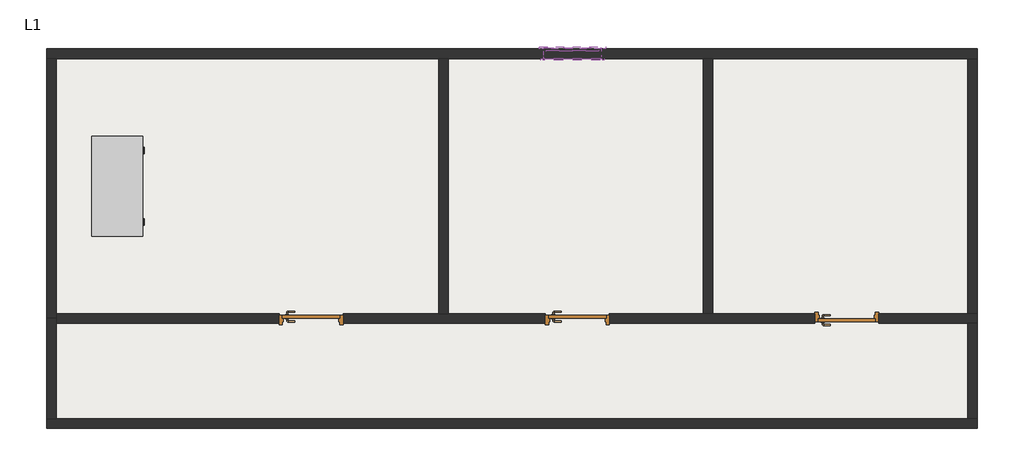
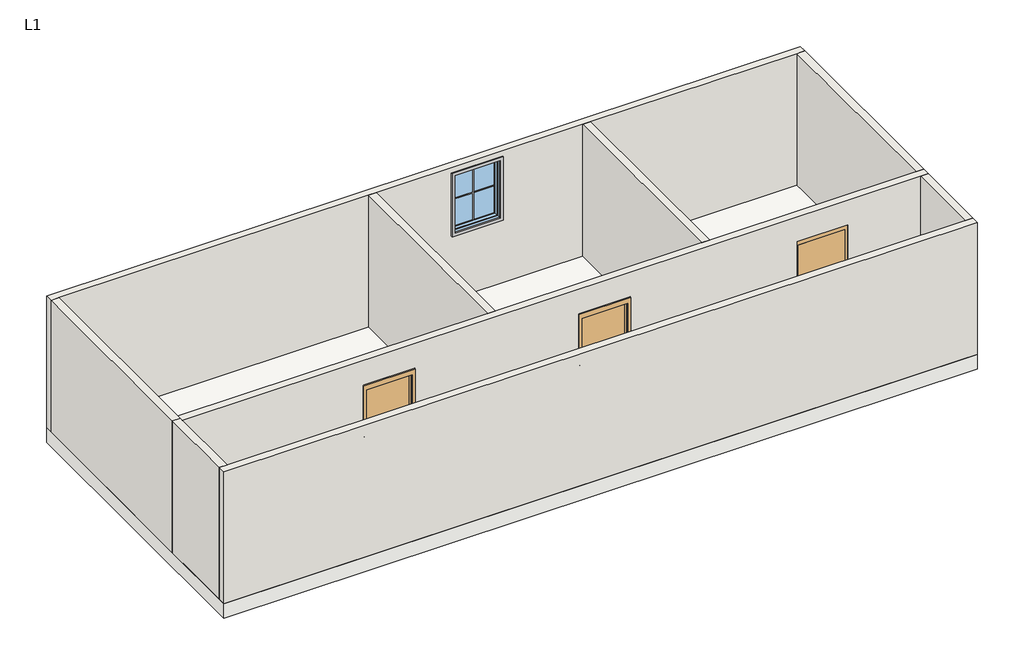
# One storey: 9 walls, 3 doors, 3 proxies, 1 furniture element, 1 slab, 1 window.
"""IFC4 building model written with IfcOpenShell, lengths in millimetres."""

import ifcopenshell
import ifcopenshell.guid

model = None  # the IFC model being written
_history = None  # IfcOwnerHistory: only IFC2X3 demands one
_inside = {}  # id of a spatial element -> (the spatial element, [elements in it])
_under = {}  # id of a project, library or spatial element -> (it, [spatial elements below it])
_declared = {}  # id of a project -> (the project, [libraries it declares])
_typed = {}  # id of a type object -> (the type object, [elements of that type])
_made_of = {}  # id of a material, layer set ... -> (it, [elements and type objects made of it])


def new_model(schema):
    """Start an empty IFC model of exactly this schema.

    Asked for "IFC4X3", IfcOpenShell would pick the latest addendum, in which some entities
    have other attributes; the version numbers below select the first issue.
    IFC2X3 requires an IfcOwnerHistory on every rooted entity: one is made here for all.
    """
    global model, _history
    if schema == "IFC4X3":
        model = ifcopenshell.file(schema_version=(4, 3, 0, 0))
    else:
        model = ifcopenshell.file(schema=schema)
    _inside.clear()
    _under.clear()
    _declared.clear()
    _typed.clear()
    _made_of.clear()
    _history = None
    if model.schema == "IFC2X3":
        org = make("IfcOrganization", Name="unknown")
        user = make(
            "IfcPersonAndOrganization",
            ThePerson=make("IfcPerson", FamilyName="unknown"),
            TheOrganization=org,
        )
        app = make(
            "IfcApplication",
            ApplicationDeveloper=org,
            Version="unknown",
            ApplicationFullName="unknown",
            ApplicationIdentifier="unknown",
        )
        _history = make(
            "IfcOwnerHistory",
            OwningUser=user,
            OwningApplication=app,
            ChangeAction="ADDED",
            CreationDate=0,
        )
    return model


def make(cls, **values):
    """One entity of the class cls with the attributes given. An attribute that is None is left unset."""
    return model.create_entity(
        cls, **{name: value for name, value in values.items() if value is not None}
    )


def rooted(cls, **values):
    """An entity with a GlobalId (a new one), such as an element, a storey or a relation."""
    return make(cls, GlobalId=ifcopenshell.guid.new(), OwnerHistory=_history, **values)


def si_unit(unit_type, name, prefix=None):
    """IfcSIUnit, for example si_unit("LENGTHUNIT", "METRE", prefix="MILLI")."""
    return make("IfcSIUnit", UnitType=unit_type, Prefix=prefix, Name=name)


def assignment(units):
    """IfcUnitAssignment: the units of a project."""
    return None if units is None else make("IfcUnitAssignment", Units=units)


def point(xyz):
    """IfcCartesianPoint."""
    return None if xyz is None else make("IfcCartesianPoint", Coordinates=xyz)


def direction(xyz):
    """IfcDirection."""
    return None if xyz is None else make("IfcDirection", DirectionRatios=xyz)


def frame(location, z_axis=None, x_axis=None):
    """IfcAxis2Placement3D, a coordinate frame: its origin and axes. An axis left out is left unset."""
    return make(
        "IfcAxis2Placement3D",
        Location=point(location),
        Axis=direction(z_axis),
        RefDirection=direction(x_axis),
    )


def frame_2d(location, x_axis=None):
    """IfcAxis2Placement2D, a coordinate frame in the plane: its origin and x axis."""
    return make(
        "IfcAxis2Placement2D", Location=point(location), RefDirection=direction(x_axis)
    )


def origin():
    """The frame at (0, 0, 0) with its axes left unset."""
    return frame((0.0, 0.0, 0.0))


def origin_with_axes():
    """The frame at (0, 0, 0) with the z axis (0, 0, 1) and the x axis (1, 0, 0) written out."""
    return frame((0.0, 0.0, 0.0), z_axis=(0.0, 0.0, 1.0), x_axis=(1.0, 0.0, 0.0))


def place(relative_to, where):
    """IfcLocalPlacement: puts the frame where relative to a parent placement (None: the world)."""
    return make(
        "IfcLocalPlacement", PlacementRelTo=relative_to, RelativePlacement=where
    )


def context(
    kind, dimensions, precision=None, world=None, true_north=None, identifier=None
):
    """IfcGeometricRepresentationContext, for example the 3D "Model" context."""
    return make(
        "IfcGeometricRepresentationContext",
        ContextIdentifier=identifier,
        ContextType=kind,
        CoordinateSpaceDimension=dimensions,
        Precision=precision,
        WorldCoordinateSystem=world,
        TrueNorth=true_north,
    )


def project(units=None, contexts=None):
    """IfcProject with its units and contexts."""
    return rooted(
        "IfcProject",
        Name="project",
        RepresentationContexts=contexts,
        UnitsInContext=assignment(units),
    )


def spatial(cls, under=None, at=None, **own):
    """A site, building, storey or space (cls), placed at a placement, below another one or the project."""
    s = rooted(cls, ObjectPlacement=at, **own)
    if under is not None:
        _under.setdefault(under.id(), (under, []))[1].append(s)
    return s


def polyline(points):
    """IfcPolyline through the points."""
    return make("IfcPolyline", Points=[point(p) for p in points])


def circle_curve(where, radius):
    """IfcCircle in the frame where."""
    return make("IfcCircle", Position=where, Radius=radius)


def ellipse_curve(where, semi_axis1, semi_axis2):
    """IfcEllipse in the frame where."""
    return make(
        "IfcEllipse", Position=where, SemiAxis1=semi_axis1, SemiAxis2=semi_axis2
    )


def trimmed(basis, trim1, trim2, sense, master):
    """IfcTrimmedCurve: the piece of a basis curve between two trims."""
    return make(
        "IfcTrimmedCurve",
        BasisCurve=basis,
        Trim1=trim1,
        Trim2=trim2,
        SenseAgreement=sense,
        MasterRepresentation=master,
    )


def segment(curve, same_sense, transition):
    """IfcCompositeCurveSegment."""
    return make(
        "IfcCompositeCurveSegment",
        Transition=transition,
        SameSense=same_sense,
        ParentCurve=curve,
    )


def composite_curve(segments, self_intersect=None):
    """IfcCompositeCurve: segments joined end to end."""
    return make("IfcCompositeCurve", Segments=segments, SelfIntersect=self_intersect)


def outline(outer, holes=None, kind="AREA"):
    """IfcArbitraryClosedProfileDef: a profile drawn as a closed curve; with holes, ...WithVoids."""
    if holes is None:
        return make("IfcArbitraryClosedProfileDef", ProfileType=kind, OuterCurve=outer)
    return make(
        "IfcArbitraryProfileDefWithVoids",
        ProfileType=kind,
        OuterCurve=outer,
        InnerCurves=holes,
    )


def extrude(swept, where, along, depth):
    """IfcExtrudedAreaSolid: the profile swept, set in the frame where, extruded along a direction by depth."""
    return make(
        "IfcExtrudedAreaSolid",
        SweptArea=swept,
        Position=where,
        ExtrudedDirection=direction(along),
        Depth=depth,
    )


def faces_of(points, faces, orient=None, outer=None):
    """IfcFace entities. A face is a list of loops; a loop is a list of indices into points, from 0.

    orient and outer hold one flag for each loop. By default every Orientation is true, the
    first loop of a face is its IfcFaceOuterBound and the others are IfcFaceBound.
    """
    made = []
    for i, loops in enumerate(faces):
        bounds = []
        for j, loop in enumerate(loops):
            is_outer = j == 0 if outer is None else outer[i][j]
            bounds.append(
                make(
                    "IfcFaceOuterBound" if is_outer else "IfcFaceBound",
                    Bound=make("IfcPolyLoop", Polygon=[points[k] for k in loop]),
                    Orientation=True if orient is None else orient[i][j],
                )
            )
        made.append(make("IfcFace", Bounds=bounds))
    return made


def faceted_brep(points, faces, orient=None, outer=None, voids=None):
    """IfcFacetedBrep: a solid bounded by flat faces; with voids (closed shells), ...WithVoids."""
    shared = [point(p) for p in points]
    hull = make("IfcClosedShell", CfsFaces=faces_of(shared, faces, orient, outer))
    if voids is None:
        return make("IfcFacetedBrep", Outer=hull)
    return make(
        "IfcFacetedBrepWithVoids",
        Outer=hull,
        Voids=[
            make(cls, CfsFaces=faces_of(shared, fs, o, b)) for cls, fs, o, b in voids
        ],
    )


def shape(context_of_items, identifier, shape_type, items):
    """IfcShapeRepresentation: the items that make up one representation, for example the "Body"."""
    return make(
        "IfcShapeRepresentation",
        ContextOfItems=context_of_items,
        RepresentationIdentifier=identifier,
        RepresentationType=shape_type,
        Items=items,
    )


def source(mapping_origin, context_of_items, identifier, shape_type, items):
    """IfcRepresentationMap: a shape defined once, which mapped items show again and again."""
    return make(
        "IfcRepresentationMap",
        MappingOrigin=mapping_origin,
        MappedRepresentation=shape(context_of_items, identifier, shape_type, items),
    )


def transform(
    local_origin,
    x_axis=None,
    y_axis=None,
    z_axis=None,
    scale=None,
    scale2=None,
    scale3=None,
    uniform=True,
):
    """IfcCartesianTransformationOperator3D, or its non-uniform kind. x_axis, y_axis, z_axis: its Axis1, 2, 3."""
    if uniform:
        return make(
            "IfcCartesianTransformationOperator3D",
            Axis1=direction(x_axis),
            Axis2=direction(y_axis),
            LocalOrigin=point(local_origin),
            Scale=scale,
            Axis3=direction(z_axis),
        )
    return make(
        "IfcCartesianTransformationOperator3DnonUniform",
        Axis1=direction(x_axis),
        Axis2=direction(y_axis),
        LocalOrigin=point(local_origin),
        Scale=scale,
        Axis3=direction(z_axis),
        Scale2=scale2,
        Scale3=scale3,
    )


def mapped(mapping_source, mapping_target):
    """IfcMappedItem: shows the shape of a source again, moved by a transform."""
    return make(
        "IfcMappedItem", MappingSource=mapping_source, MappingTarget=mapping_target
    )


def made_of(thing, what):
    """Note that an element or type object is made of a material, layer set ...; save() writes the relation."""
    if what is not None:
        _made_of.setdefault(what.id(), (what, []))[1].append(thing)
    return thing


def element(
    cls,
    number,
    at=None,
    inside=None,
    cuts=None,
    type_object=None,
    material=None,
    context=None,
    identifier="Body",
    shape_type=None,
    held_by="IfcProductDefinitionShape",
    body=None,
    shapes=None,
    **own,
):
    """One element of the class cls, such as IfcWall. Its Tag is "e" and its number.

    at: its placement. inside: the storey or other place that contains it. cuts: it is an
    opening in that element (IfcRelVoidsElement). A single representation is given by context,
    identifier, shape_type and body (its items); several are given by shapes. held_by: the class
    of the entity that holds the representations. save() writes the other relations.
    """
    e = rooted(cls, Tag="e%d" % number, ObjectPlacement=at, **own)
    if body is not None:
        shapes = [shape(context, identifier, shape_type, body)]
    if shapes is not None:
        e.Representation = make(held_by, Representations=shapes)
    if inside is not None:
        _inside.setdefault(inside.id(), (inside, []))[1].append(e)
    if cuts is not None:
        rooted(
            "IfcRelVoidsElement", RelatingBuildingElement=cuts, RelatedOpeningElement=e
        )
    if type_object is not None:
        _typed.setdefault(type_object.id(), (type_object, []))[1].append(e)
    return made_of(e, material)


def aggregate(whole, parts):
    """IfcRelAggregates: a whole, such as a stair, and the parts it consists of."""
    return rooted("IfcRelAggregates", RelatingObject=whole, RelatedObjects=parts)


def save(model, path):
    """Write the relations noted so far, then the file.

    IfcRelAggregates (storeys below a building ...), IfcRelContainedInSpatialStructure (elements
    in a storey), IfcRelDefinesByType, IfcRelAssociatesMaterial and IfcRelDeclares: one each for
    every whole, place, type object, material and project.
    """
    for whole, parts in _under.values():
        aggregate(whole, parts)
    for where, things in _inside.values():
        rooted(
            "IfcRelContainedInSpatialStructure",
            RelatedElements=things,
            RelatingStructure=where,
        )
    for kind, things in _typed.values():
        rooted("IfcRelDefinesByType", RelatedObjects=things, RelatingType=kind)
    for what, things in _made_of.values():
        rooted("IfcRelAssociatesMaterial", RelatedObjects=things, RelatingMaterial=what)
    for by, libraries in _declared.values():
        rooted("IfcRelDeclares", RelatingContext=by, RelatedDefinitions=libraries)
    model.write(path)


def plane_surface(at):
    """IfcPlane: the flat surface through the origin of the frame at, square to its z axis."""
    return make("IfcPlane", Position=at)


def cylinder_surface(at, radius):
    """IfcCylindricalSurface: all points at the distance radius from the z axis of the frame at."""
    return make("IfcCylindricalSurface", Position=at, Radius=radius)


def revolved_surface(curve, axis_point, axis_direction):
    """IfcSurfaceOfRevolution: the curve turned about the line through axis_point along axis_direction."""
    return make(
        "IfcSurfaceOfRevolution",
        SweptCurve=make("IfcArbitraryOpenProfileDef", ProfileType="CURVE", Curve=curve),
        AxisPosition=make("IfcAxis1Placement", Location=point(axis_point), Axis=direction(axis_direction)),
    )


def advanced_brep(points, edges, surfaces, faces):
    """IfcAdvancedBrep: a solid bounded by faces that lie on surfaces and meet in shared edges.

    An edge is (start, end): straight between two places in points (the first is 0);
    or (start, end, curve); or (start, end, curve, False) where it runs against its curve.
    A face is (place in surfaces, loops), or (place, loops, False) where it looks against
    its surface's normal. A loop lists edges by number (the first is 1), with a minus sign
    where the edge is run from its end to its start. The first loop is the outer one.
    """
    corners = [point(p) for p in points]
    vertices = [make("IfcVertexPoint", VertexGeometry=c) for c in corners]
    made = []
    for start, end, *more in edges:
        made.append(
            make(
                "IfcEdgeCurve",
                EdgeStart=vertices[start],
                EdgeEnd=vertices[end],
                EdgeGeometry=more[0] if more else make("IfcPolyline", Points=[corners[start], corners[end]]),
                SameSense=more[1] if len(more) > 1 else True,
            )
        )
    hull = []
    for where, loops, *sense in faces:
        bounds = []
        for j, loop in enumerate(loops):
            ring = [make("IfcOrientedEdge", EdgeElement=made[abs(k) - 1], Orientation=k > 0) for k in loop]
            bounds.append(
                make(
                    "IfcFaceOuterBound" if j == 0 else "IfcFaceBound",
                    Bound=make("IfcEdgeLoop", EdgeList=ring),
                    Orientation=True,
                )
            )
        hull.append(make("IfcAdvancedFace", Bounds=bounds, FaceSurface=surfaces[where], SameSense=sense[0] if sense else True))
    return make("IfcAdvancedBrep", Outer=make("IfcClosedShell", CfsFaces=hull))


def m_muntin_pattern_2x2_m_muntin_pattern_2x2_ad852c99(model_context):
    return source(origin(), model_context, "Body", "SweptSolid", [
        extrude(outline(polyline([(568.25, -6.35), (568.25, -411.9), (555.55, -411.9), (555.55, -6.35), (0.0, -6.35), (0.0, 6.35), (555.55, 6.35), (555.55, 411.9), (568.25, 411.9), (568.25, 6.35), (1123.8, 6.35), (1123.8, -6.35), (568.25, -6.35)])), frame((0.0, -22.225, 0.0), z_axis=(0.0, 1.0, 0.0), x_axis=(0.0, 0.0, 1.0)), (0.0, 0.0, 1.0), 12.7),
        extrude(outline(polyline([(568.25, -6.35), (568.25, -411.9), (555.55, -411.9), (555.55, -6.35), (0.0, -6.35), (0.0, 6.35), (555.55, 6.35), (555.55, 411.9), (568.25, 411.9), (568.25, 6.35), (1123.8, 6.35), (1123.8, -6.35), (568.25, -6.35)])), frame((0.0, 9.525, 0.0), z_axis=(0.0, 1.0, 0.0), x_axis=(0.0, 0.0, 1.0)), (0.0, 0.0, 1.0), 12.7),
    ])


def m_trim_window_exterior_flat_with_sill_71544b40(model_context):
    return source(origin(), model_context, "Body", "SweptSolid", [
        extrude(outline(polyline([(510.0, -1220.4323709), (510.0, -1280.4323709), (-510.0, -1280.4323709), (-510.0, -1220.4323709), (510.0, -1220.4323709)])), origin_with_axes(), (0.0, 0.0, 1.0), 19.05),
        extrude(outline(polyline([(-1230.0, 38.1), (-1202.4580645, 38.1), (-1200.0, 19.05), (-1200.0, 0.0), (-1220.4323709, 0.0), (-1220.4323709, 19.05), (-1230.0, 19.05), (-1230.0, 38.1)])), frame((-522.7, 0.0, 0.0), z_axis=(1.0, 0.0, 0.0), x_axis=(0.0, 1.0, 0.0)), (0.0, 0.0, 1.0), 1045.4),
        extrude(outline(polyline([(-510.0, 60.0), (510.0, 60.0), (510.0, -1200.0), (450.0, -1200.0), (450.0, 0.0), (-450.0, 0.0), (-450.0, -1200.0), (-510.0, -1200.0), (-510.0, 60.0)])), origin_with_axes(), (0.0, 0.0, 1.0), 19.05),
    ])


def m_trim_window_interior_flat_picture_frame_24fe8ef8(model_context):
    return source(origin(), model_context, "Body", "SweptSolid", [
        extrude(outline(polyline([(497.3, 47.3), (497.3, -1247.3), (-497.3, -1247.3), (-497.3, 47.3), (497.3, 47.3)]), holes=[polyline([(437.3, -12.7), (-437.3, -12.7), (-437.3, -1187.3), (437.3, -1187.3), (437.3, -12.7)])]), origin_with_axes(), (0.0, 0.0, 1.0), 30.0),
    ])


def m_door_passage_single_flush_900_x_2100mm_f70d95c9(model_context):
    return source(origin(), model_context, "Body", "SolidModel", [
        advanced_brep(
        [(-384.990625, 3.35, 1000.0), (-364.990625, 3.35, 1000.0), (-364.990625, -26.65, 1000.0), (-384.990625, -26.65, 1000.0), (-359.990625, -31.65, 1000.0), (-359.990625, -51.65, 1000.0), (-254.990625, -51.65, 1000.0), (-254.990625, -31.65, 1000.0)],
        [
            (0, 1, circle_curve(frame((-374.990625, 3.35, 1000.0), z_axis=(0.0, 1.0, 0.0), x_axis=(1.0, 0.0, 0.0)), 10.0)),
            (1, 0, circle_curve(frame((-374.990625, 3.35, 1000.0), z_axis=(0.0, 1.0, 0.0), x_axis=(1.0, 0.0, 0.0)), 10.0)),
            (1, 2),
            (2, 3, circle_curve(frame((-374.990625, -26.65, 1000.0), z_axis=(0.0, 1.0, 0.0), x_axis=(1.0, 0.0, 0.0)), 10.0)),
            (3, 0),
            (3, 2, circle_curve(frame((-374.990625, -26.65, 1000.0), z_axis=(0.0, 1.0, 0.0), x_axis=(1.0, 0.0, 0.0)), 10.0)),
            (4, 5, circle_curve(frame((-359.990625, -41.65, 1000.0), z_axis=(-1.0, 0.0, 0.0), x_axis=(0.0, 1.0, 0.0)), 10.0)),
            (5, 3, circle_curve(frame((-359.990625, -26.65, 1000.0), z_axis=(0.0, 0.0, -1.0), x_axis=(-1.0, 0.0, 0.0)), 25.0)),
            (2, 4, circle_curve(frame((-359.990625, -26.65, 1000.0), z_axis=(0.0, 0.0, 1.0), x_axis=(-1.0, 0.0, 0.0)), 5.0)),
            (5, 4, circle_curve(frame((-359.990625, -41.65, 1000.0), z_axis=(-1.0, 0.0, 0.0), x_axis=(0.0, 1.0, 0.0)), 10.0)),
            (6, 7, circle_curve(frame((-254.990625, -41.65, 1000.0), z_axis=(1.0, 0.0, 0.0), x_axis=(0.0, 1.0, 0.0)), 10.0)),
            (7, 6, circle_curve(frame((-254.990625, -41.65, 1000.0), z_axis=(1.0, 0.0, 0.0), x_axis=(0.0, 1.0, 0.0)), 10.0)),
            (4, 7),
            (6, 5),
        ],
        [
            plane_surface(frame((-374.990625, 3.35, 1000.0), z_axis=(0.0, 1.0, 0.0), x_axis=(0.0, 0.0, 1.0))),
            cylinder_surface(frame((-374.990625, 3.35, 1000.0), z_axis=(0.0, 1.0, 0.0), x_axis=(1.0, 0.0, 0.0)), 10.0),
            revolved_surface(trimmed(ellipse_curve(frame((-374.990625, -26.65, 1000.0), z_axis=(0.0, -1.0, 0.0), x_axis=(1.0, 0.0, 0.0)), 10.0, 10.0), [point((-384.990625, -26.65, 1000.0))], [point((-364.990625, -26.65, 1000.0))], True, "CARTESIAN"), (-359.990625, -26.65, 1000.0), (0.0, 0.0, -1.0)),
            revolved_surface(trimmed(ellipse_curve(frame((-374.990625, -26.65, 1000.0), z_axis=(0.0, -1.0, 0.0), x_axis=(1.0, 0.0, 0.0)), 10.0, 10.0), [point((-364.990625, -26.65, 1000.0))], [point((-384.990625, -26.65, 1000.0))], True, "CARTESIAN"), (-359.990625, -26.65, 1000.0), (0.0, 0.0, -1.0)),
            plane_surface(frame((-254.990625, -41.65, 1000.0), z_axis=(1.0, 0.0, 0.0), x_axis=(0.0, 0.0, 1.0))),
            cylinder_surface(frame((-359.990625, -41.65, 1000.0), z_axis=(-1.0, 0.0, 0.0), x_axis=(0.0, 1.0, 0.0)), 10.0),
        ],
        [
            (0, [[1, 2]]),
            (1, [[3, 4, 5, -2]]),
            (1, [[-5, 6, -3, -1]]),
            (2, [[7, 8, -4, 9]]),
            (3, [[10, -9, -6, -8]]),
            (4, [[11, 12]]),
            (5, [[13, -11, 14, -7]]),
            (5, [[-14, -12, -13, -10]]),
        ],
    ),
        extrude(outline(composite_curve([segment(trimmed(circle_curve(frame_2d((1000.0, -377.490625)), 30.0), [point((1000.0, -407.490625))], [point((1000.0, -347.490625))], False, "CARTESIAN"), True, "CONTINUOUS"), segment(trimmed(circle_curve(frame_2d((1000.0, -377.490625)), 30.0), [point((1000.0, -347.490625))], [point((1000.0, -407.490625))], False, "CARTESIAN"), True, "CONTINUOUS")], self_intersect=False)), frame((0.0, 3.35, 0.0), z_axis=(0.0, 1.0, 0.0), x_axis=(0.0, 0.0, 1.0)), (0.0, 0.0, 1.0), 8.0),
        advanced_brep(
        [(-384.990625, 64.35, 1000.0), (-364.990625, 64.35, 1000.0), (-384.990625, 94.35, 1000.0), (-364.990625, 94.35, 1000.0), (-359.990625, 99.35, 1000.0), (-359.990625, 119.35, 1000.0), (-254.990625, 119.35, 1000.0), (-254.990625, 99.35, 1000.0)],
        [
            (0, 1, circle_curve(frame((-374.990625, 64.35, 1000.0), z_axis=(0.0, -1.0, 0.0), x_axis=(1.0, 0.0, 0.0)), 10.0)),
            (1, 0, circle_curve(frame((-374.990625, 64.35, 1000.0), z_axis=(0.0, -1.0, 0.0), x_axis=(1.0, 0.0, 0.0)), 10.0)),
            (0, 2),
            (2, 3, circle_curve(frame((-374.990625, 94.35, 1000.0), z_axis=(0.0, -1.0, 0.0), x_axis=(1.0, 0.0, 0.0)), 10.0)),
            (3, 1),
            (3, 2, circle_curve(frame((-374.990625, 94.35, 1000.0), z_axis=(0.0, -1.0, 0.0), x_axis=(1.0, 0.0, 0.0)), 10.0)),
            (4, 3, circle_curve(frame((-359.990625, 94.35, 1000.0), z_axis=(0.0, 0.0, 1.0), x_axis=(-1.0, 0.0, 0.0)), 5.0)),
            (2, 5, circle_curve(frame((-359.990625, 94.35, 1000.0), z_axis=(0.0, 0.0, -1.0), x_axis=(-1.0, 0.0, 0.0)), 25.0)),
            (5, 4, circle_curve(frame((-359.990625, 109.35, 1000.0), z_axis=(-1.0, 0.0, 0.0), x_axis=(0.0, -1.0, 0.0)), 10.0)),
            (4, 5, circle_curve(frame((-359.990625, 109.35, 1000.0), z_axis=(-1.0, 0.0, 0.0), x_axis=(0.0, -1.0, 0.0)), 10.0)),
            (6, 7, circle_curve(frame((-254.990625, 109.35, 1000.0), z_axis=(1.0, 0.0, 0.0), x_axis=(0.0, -1.0, 0.0)), 10.0)),
            (7, 6, circle_curve(frame((-254.990625, 109.35, 1000.0), z_axis=(1.0, 0.0, 0.0), x_axis=(0.0, -1.0, 0.0)), 10.0)),
            (5, 6),
            (7, 4),
        ],
        [
            plane_surface(frame((-374.990625, 64.35, 1000.0), z_axis=(0.0, -1.0, 0.0), x_axis=(0.0, 0.0, 1.0))),
            cylinder_surface(frame((-374.990625, 64.35, 1000.0), z_axis=(0.0, -1.0, 0.0), x_axis=(1.0, 0.0, 0.0)), 10.0),
            revolved_surface(trimmed(ellipse_curve(frame((-374.990625, 94.35, 1000.0), z_axis=(0.0, -1.0, 0.0), x_axis=(1.0, 0.0, 0.0)), 10.0, 10.0), [point((-384.990625, 94.35, 1000.0))], [point((-364.990625, 94.35, 1000.0))], True, "CARTESIAN"), (-359.990625, 94.35, 1000.0), (0.0, 0.0, -1.0)),
            revolved_surface(trimmed(ellipse_curve(frame((-374.990625, 94.35, 1000.0), z_axis=(0.0, -1.0, 0.0), x_axis=(1.0, 0.0, 0.0)), 10.0, 10.0), [point((-364.990625, 94.35, 1000.0))], [point((-384.990625, 94.35, 1000.0))], True, "CARTESIAN"), (-359.990625, 94.35, 1000.0), (0.0, 0.0, -1.0)),
            plane_surface(frame((-254.990625, 109.35, 1000.0), z_axis=(1.0, 0.0, 0.0), x_axis=(0.0, 0.0, 1.0))),
            cylinder_surface(frame((-359.990625, 109.35, 1000.0), z_axis=(-1.0, 0.0, 0.0), x_axis=(0.0, -1.0, 0.0)), 10.0),
        ],
        [
            (0, [[1, 2]]),
            (1, [[-1, 3, 4, 5]]),
            (1, [[-2, -5, 6, -3]]),
            (2, [[7, -4, 8, 9]]),
            (3, [[-8, -6, -7, 10]]),
            (4, [[11, 12]]),
            (5, [[-9, 13, -12, 14]]),
            (5, [[-10, -14, -11, -13]]),
        ],
    ),
        extrude(outline(composite_curve([segment(trimmed(circle_curve(frame_2d((1000.0, -377.490625)), 30.0), [point((1000.0, -407.490625))], [point((1000.0, -347.490625))], False, "CARTESIAN"), True, "CONTINUOUS"), segment(trimmed(circle_curve(frame_2d((1000.0, -377.490625)), 30.0), [point((1000.0, -347.490625))], [point((1000.0, -407.490625))], False, "CARTESIAN"), True, "CONTINUOUS")], self_intersect=False)), frame((0.0, 56.35, 0.0), z_axis=(0.0, 1.0, 0.0), x_axis=(0.0, 0.0, 1.0)), (0.0, 0.0, 1.0), 8.0),
        extrude(outline(polyline([(450.0, 11.35), (-450.0, 11.35), (-450.0, 56.35), (450.0, 56.35), (450.0, 11.35)])), origin_with_axes(), (0.0, 0.0, 1.0), 2100.0),
        faceted_brep([(450.0, 6.5875, 0.0), (450.0, 56.35, 0.0), (500.0, 56.35, 0.0), (500.0, -93.65, 0.0), (450.0, -93.65, 0.0), (450.0, -44.4375, 0.0), (434.125, -44.4375, 0.0), (434.125, 6.5875, 0.0), (450.0, 6.5875, 2100.0), (450.0, 56.35, 2100.0), (-450.0, 56.35, 2100.0), (-450.0, 56.35, 0.0), (-500.0, 56.35, 0.0), (-500.0, 56.35, 2200.0), (500.0, 56.35, 2200.0), (500.0, -93.65, 2200.0), (-500.0, -93.65, 2200.0), (-500.0, -93.65, 0.0), (-450.0, -93.65, 0.0), (-450.0, -93.65, 2100.0), (450.0, -93.65, 2100.0), (450.0, -44.4375, 2100.0), (-450.0, -44.4375, 2100.0), (-450.0, -44.4375, 0.0), (-434.125, -44.4375, 0.0), (-434.125, -44.4375, 2084.125), (434.125, -44.4375, 2084.125), (434.125, 6.5875, 2084.125), (-434.125, 6.5875, 2084.125), (-434.125, 6.5875, 0.0), (-450.0, 6.5875, 0.0), (-450.0, 6.5875, 2100.0)], [[[0, 1, 2, 3, 4, 5, 6, 7]], [[1, 0, 8, 9]], [[2, 1, 9, 10, 11, 12, 13, 14]], [[3, 2, 14, 15]], [[4, 3, 15, 16, 17, 18, 19, 20]], [[5, 4, 20, 21]], [[6, 5, 21, 22, 23, 24, 25, 26]], [[7, 6, 26, 27]], [[0, 7, 27, 28, 29, 30, 31, 8]], [[9, 8, 31, 10]], [[20, 19, 22, 21]], [[26, 25, 28, 27]], [[12, 11, 30, 29, 24, 23, 18, 17]], [[11, 10, 31, 30]], [[13, 12, 17, 16]], [[19, 18, 23, 22]], [[25, 24, 29, 28]], [[15, 14, 13, 16]]]),
    ])


def m_door_passage_single_flush_900_x_2100mm_89322b7b(model_context):
    return source(origin(), model_context, "Body", "SolidModel", [
        advanced_brep(
        [(-384.990625, -3.35, 1000.0), (-364.990625, -3.35, 1000.0), (-384.990625, 26.65, 1000.0), (-364.990625, 26.65, 1000.0), (-359.990625, 31.65, 1000.0), (-359.990625, 51.65, 1000.0), (-254.990625, 51.65, 1000.0), (-254.990625, 31.65, 1000.0)],
        [
            (0, 1, circle_curve(frame((-374.990625, -3.35, 1000.0), z_axis=(0.0, -1.0, 0.0), x_axis=(1.0, 0.0, 0.0)), 10.0)),
            (1, 0, circle_curve(frame((-374.990625, -3.35, 1000.0), z_axis=(0.0, -1.0, 0.0), x_axis=(1.0, 0.0, 0.0)), 10.0)),
            (0, 2),
            (2, 3, circle_curve(frame((-374.990625, 26.65, 1000.0), z_axis=(0.0, -1.0, 0.0), x_axis=(1.0, 0.0, 0.0)), 10.0)),
            (3, 1),
            (3, 2, circle_curve(frame((-374.990625, 26.65, 1000.0), z_axis=(0.0, -1.0, 0.0), x_axis=(1.0, 0.0, 0.0)), 10.0)),
            (4, 3, circle_curve(frame((-359.990625, 26.65, 1000.0), z_axis=(0.0, 0.0, 1.0), x_axis=(-1.0, 0.0, 0.0)), 5.0)),
            (2, 5, circle_curve(frame((-359.990625, 26.65, 1000.0), z_axis=(0.0, 0.0, -1.0), x_axis=(-1.0, 0.0, 0.0)), 25.0)),
            (5, 4, circle_curve(frame((-359.990625, 41.65, 1000.0), z_axis=(-1.0, 0.0, 0.0), x_axis=(0.0, -1.0, 0.0)), 10.0)),
            (4, 5, circle_curve(frame((-359.990625, 41.65, 1000.0), z_axis=(-1.0, 0.0, 0.0), x_axis=(0.0, -1.0, 0.0)), 10.0)),
            (6, 7, circle_curve(frame((-254.990625, 41.65, 1000.0), z_axis=(1.0, 0.0, 0.0), x_axis=(0.0, -1.0, 0.0)), 10.0)),
            (7, 6, circle_curve(frame((-254.990625, 41.65, 1000.0), z_axis=(1.0, 0.0, 0.0), x_axis=(0.0, -1.0, 0.0)), 10.0)),
            (5, 6),
            (7, 4),
        ],
        [
            plane_surface(frame((-374.990625, -3.35, 1000.0), z_axis=(0.0, -1.0, 0.0), x_axis=(0.0, 0.0, 1.0))),
            cylinder_surface(frame((-374.990625, -3.35, 1000.0), z_axis=(0.0, -1.0, 0.0), x_axis=(1.0, 0.0, 0.0)), 10.0),
            revolved_surface(trimmed(ellipse_curve(frame((-374.990625, 26.65, 1000.0), z_axis=(0.0, -1.0, 0.0), x_axis=(1.0, 0.0, 0.0)), 10.0, 10.0), [point((-384.990625, 26.65, 1000.0))], [point((-364.990625, 26.65, 1000.0))], True, "CARTESIAN"), (-359.990625, 26.65, 1000.0), (0.0, 0.0, -1.0)),
            revolved_surface(trimmed(ellipse_curve(frame((-374.990625, 26.65, 1000.0), z_axis=(0.0, -1.0, 0.0), x_axis=(1.0, 0.0, 0.0)), 10.0, 10.0), [point((-364.990625, 26.65, 1000.0))], [point((-384.990625, 26.65, 1000.0))], True, "CARTESIAN"), (-359.990625, 26.65, 1000.0), (0.0, 0.0, -1.0)),
            plane_surface(frame((-254.990625, 41.65, 1000.0), z_axis=(1.0, 0.0, 0.0), x_axis=(0.0, 0.0, 1.0))),
            cylinder_surface(frame((-359.990625, 41.65, 1000.0), z_axis=(-1.0, 0.0, 0.0), x_axis=(0.0, -1.0, 0.0)), 10.0),
        ],
        [
            (0, [[1, 2]]),
            (1, [[-1, 3, 4, 5]]),
            (1, [[-2, -5, 6, -3]]),
            (2, [[7, -4, 8, 9]]),
            (3, [[-8, -6, -7, 10]]),
            (4, [[11, 12]]),
            (5, [[-9, 13, -12, 14]]),
            (5, [[-10, -14, -11, -13]]),
        ],
    ),
        extrude(outline(composite_curve([segment(trimmed(circle_curve(frame_2d((1000.0, -377.490625)), 30.0), [point((1000.0, -407.490625))], [point((1000.0, -347.490625))], False, "CARTESIAN"), True, "CONTINUOUS"), segment(trimmed(circle_curve(frame_2d((1000.0, -377.490625)), 30.0), [point((1000.0, -347.490625))], [point((1000.0, -407.490625))], False, "CARTESIAN"), True, "CONTINUOUS")], self_intersect=False)), frame((0.0, -11.35, 0.0), z_axis=(0.0, 1.0, 0.0), x_axis=(0.0, 0.0, 1.0)), (0.0, 0.0, 1.0), 8.0),
        advanced_brep(
        [(-384.990625, -64.35, 1000.0), (-364.990625, -64.35, 1000.0), (-364.990625, -94.35, 1000.0), (-384.990625, -94.35, 1000.0), (-359.990625, -99.35, 1000.0), (-359.990625, -119.35, 1000.0), (-254.990625, -119.35, 1000.0), (-254.990625, -99.35, 1000.0)],
        [
            (0, 1, circle_curve(frame((-374.990625, -64.35, 1000.0), z_axis=(0.0, 1.0, 0.0), x_axis=(1.0, 0.0, 0.0)), 10.0)),
            (1, 0, circle_curve(frame((-374.990625, -64.35, 1000.0), z_axis=(0.0, 1.0, 0.0), x_axis=(1.0, 0.0, 0.0)), 10.0)),
            (1, 2),
            (2, 3, circle_curve(frame((-374.990625, -94.35, 1000.0), z_axis=(0.0, 1.0, 0.0), x_axis=(1.0, 0.0, 0.0)), 10.0)),
            (3, 0),
            (3, 2, circle_curve(frame((-374.990625, -94.35, 1000.0), z_axis=(0.0, 1.0, 0.0), x_axis=(1.0, 0.0, 0.0)), 10.0)),
            (4, 5, circle_curve(frame((-359.990625, -109.35, 1000.0), z_axis=(-1.0, 0.0, 0.0), x_axis=(0.0, 1.0, 0.0)), 10.0)),
            (5, 3, circle_curve(frame((-359.990625, -94.35, 1000.0), z_axis=(0.0, 0.0, -1.0), x_axis=(-1.0, 0.0, 0.0)), 25.0)),
            (2, 4, circle_curve(frame((-359.990625, -94.35, 1000.0), z_axis=(0.0, 0.0, 1.0), x_axis=(-1.0, 0.0, 0.0)), 5.0)),
            (5, 4, circle_curve(frame((-359.990625, -109.35, 1000.0), z_axis=(-1.0, 0.0, 0.0), x_axis=(0.0, 1.0, 0.0)), 10.0)),
            (6, 7, circle_curve(frame((-254.990625, -109.35, 1000.0), z_axis=(1.0, 0.0, 0.0), x_axis=(0.0, 1.0, 0.0)), 10.0)),
            (7, 6, circle_curve(frame((-254.990625, -109.35, 1000.0), z_axis=(1.0, 0.0, 0.0), x_axis=(0.0, 1.0, 0.0)), 10.0)),
            (4, 7),
            (6, 5),
        ],
        [
            plane_surface(frame((-374.990625, -64.35, 1000.0), z_axis=(0.0, 1.0, 0.0), x_axis=(0.0, 0.0, 1.0))),
            cylinder_surface(frame((-374.990625, -64.35, 1000.0), z_axis=(0.0, 1.0, 0.0), x_axis=(1.0, 0.0, 0.0)), 10.0),
            revolved_surface(trimmed(ellipse_curve(frame((-374.990625, -94.35, 1000.0), z_axis=(0.0, -1.0, 0.0), x_axis=(1.0, 0.0, 0.0)), 10.0, 10.0), [point((-384.990625, -94.35, 1000.0))], [point((-364.990625, -94.35, 1000.0))], True, "CARTESIAN"), (-359.990625, -94.35, 1000.0), (0.0, 0.0, -1.0)),
            revolved_surface(trimmed(ellipse_curve(frame((-374.990625, -94.35, 1000.0), z_axis=(0.0, -1.0, 0.0), x_axis=(1.0, 0.0, 0.0)), 10.0, 10.0), [point((-364.990625, -94.35, 1000.0))], [point((-384.990625, -94.35, 1000.0))], True, "CARTESIAN"), (-359.990625, -94.35, 1000.0), (0.0, 0.0, -1.0)),
            plane_surface(frame((-254.990625, -109.35, 1000.0), z_axis=(1.0, 0.0, 0.0), x_axis=(0.0, 0.0, 1.0))),
            cylinder_surface(frame((-359.990625, -109.35, 1000.0), z_axis=(-1.0, 0.0, 0.0), x_axis=(0.0, 1.0, 0.0)), 10.0),
        ],
        [
            (0, [[1, 2]]),
            (1, [[3, 4, 5, -2]]),
            (1, [[-5, 6, -3, -1]]),
            (2, [[7, 8, -4, 9]]),
            (3, [[10, -9, -6, -8]]),
            (4, [[11, 12]]),
            (5, [[13, -11, 14, -7]]),
            (5, [[-14, -12, -13, -10]]),
        ],
    ),
        extrude(outline(composite_curve([segment(trimmed(circle_curve(frame_2d((1000.0, -377.490625)), 30.0), [point((1000.0, -407.490625))], [point((1000.0, -347.490625))], False, "CARTESIAN"), True, "CONTINUOUS"), segment(trimmed(circle_curve(frame_2d((1000.0, -377.490625)), 30.0), [point((1000.0, -347.490625))], [point((1000.0, -407.490625))], False, "CARTESIAN"), True, "CONTINUOUS")], self_intersect=False)), frame((0.0, -64.35, 0.0), z_axis=(0.0, 1.0, 0.0), x_axis=(0.0, 0.0, 1.0)), (0.0, 0.0, 1.0), 8.0),
        extrude(outline(polyline([(450.0, -11.35), (450.0, -56.35), (-450.0, -56.35), (-450.0, -11.35), (450.0, -11.35)])), origin_with_axes(), (0.0, 0.0, 1.0), 2100.0),
        faceted_brep([(450.0, -6.5875, 0.0), (434.125, -6.5875, 0.0), (434.125, 44.4375, 0.0), (450.0, 44.4375, 0.0), (450.0, 93.65, 0.0), (500.0, 93.65, 0.0), (500.0, -56.35, 0.0), (450.0, -56.35, 0.0), (450.0, -56.35, 2100.0), (450.0, -6.5875, 2100.0), (500.0, -56.35, 2200.0), (-500.0, -56.35, 2200.0), (-500.0, -56.35, 0.0), (-450.0, -56.35, 0.0), (-450.0, -56.35, 2100.0), (500.0, 93.65, 2200.0), (450.0, 93.65, 2100.0), (-450.0, 93.65, 2100.0), (-450.0, 93.65, 0.0), (-500.0, 93.65, 0.0), (-500.0, 93.65, 2200.0), (450.0, 44.4375, 2100.0), (434.125, 44.4375, 2084.125), (-434.125, 44.4375, 2084.125), (-434.125, 44.4375, 0.0), (-450.0, 44.4375, 0.0), (-450.0, 44.4375, 2100.0), (434.125, -6.5875, 2084.125), (-450.0, -6.5875, 2100.0), (-450.0, -6.5875, 0.0), (-434.125, -6.5875, 0.0), (-434.125, -6.5875, 2084.125)], [[[0, 1, 2, 3, 4, 5, 6, 7]], [[7, 8, 9, 0]], [[6, 10, 11, 12, 13, 14, 8, 7]], [[5, 15, 10, 6]], [[4, 16, 17, 18, 19, 20, 15, 5]], [[3, 21, 16, 4]], [[2, 22, 23, 24, 25, 26, 21, 3]], [[1, 27, 22, 2]], [[0, 9, 28, 29, 30, 31, 27, 1]], [[8, 14, 28, 9]], [[16, 21, 26, 17]], [[22, 27, 31, 23]], [[12, 19, 18, 25, 24, 30, 29, 13]], [[13, 29, 28, 14]], [[11, 20, 19, 12]], [[17, 26, 25, 18]], [[23, 31, 30, 24]], [[15, 20, 11, 10]]]),
    ])


def m_desk_1525_x_762mm_student_34485ced(model_context):
    return source(origin(), model_context, "Body", "SolidModel", [
        extrude(outline(polyline([(1118.1, 0.0), (1118.1, 635.0), (405.9, 635.0), (405.9, 0.0), (-0.5, 0.0), (-0.5, 762.0), (1524.5, 762.0), (1524.5, 0.0), (1118.1, 0.0)])), frame((0.0, 0.0, 152.0), z_axis=(0.0, 0.0, 1.0), x_axis=(1.0, 0.0, 0.0)), (0.0, 0.0, 1.0), 571.9),
        extrude(outline(polyline([(-19.55, -19.05), (-19.55, 781.05), (1543.55, 781.05), (1543.55, -19.05), (-19.55, -19.05)])), frame((0.0, 0.0, 723.9), z_axis=(0.0, 0.0, 1.0), x_axis=(1.0, 0.0, 0.0)), (0.0, 0.0, 1.0), 38.1),
        faceted_brep([(1422.9, 0.0, 152.0), (1524.5, 0.0, 152.0), (1524.5, 101.6, 152.0), (1422.9, 101.6, 152.0), (1448.3, 0.0, 0.0), (1448.3, 76.2, 0.0), (1524.5, 76.2, 0.0), (1524.5, 0.0, 0.0)], [[[0, 1, 2, 3]], [[4, 5, 6, 7]], [[4, 7, 1, 0]], [[7, 6, 2, 1]], [[6, 5, 3, 2]], [[5, 4, 0, 3]]]),
        faceted_brep([(1422.9, 762.0, 152.0), (1422.9, 660.4, 152.0), (1524.5, 660.4, 152.0), (1524.5, 762.0, 152.0), (1448.3, 762.0, 0.0), (1524.5, 762.0, 0.0), (1524.5, 685.8, 0.0), (1448.3, 685.8, 0.0)], [[[0, 1, 2, 3]], [[4, 5, 6, 7]], [[4, 7, 1, 0]], [[7, 6, 2, 1]], [[6, 5, 3, 2]], [[5, 4, 0, 3]]]),
        faceted_brep([(101.1, 762.0, 152.0), (-0.5, 762.0, 152.0), (-0.5, 660.4, 152.0), (101.1, 660.4, 152.0), (75.7, 762.0, 0.0), (75.7, 685.8, 0.0), (-0.5, 685.8, 0.0), (-0.5, 762.0, 0.0)], [[[0, 1, 2, 3]], [[4, 5, 6, 7]], [[4, 7, 1, 0]], [[7, 6, 2, 1]], [[6, 5, 3, 2]], [[5, 4, 0, 3]]]),
        faceted_brep([(101.1, 0.0, 152.0), (101.1, 101.6, 152.0), (-0.5, 101.6, 152.0), (-0.5, 0.0, 152.0), (75.7, 0.0, 0.0), (-0.5, 0.0, 0.0), (-0.5, 76.2, 0.0), (75.7, 76.2, 0.0)], [[[0, 1, 2, 3]], [[4, 5, 6, 7]], [[4, 7, 1, 0]], [[7, 6, 2, 1]], [[6, 5, 3, 2]], [[5, 4, 0, 3]]]),
        extrude(outline(polyline([(1137.15, 0.0), (1505.45, 0.0), (1505.45, -12.7), (1137.15, -12.7), (1137.15, 0.0)])), frame((0.0, 0.0, 602.85), z_axis=(0.0, 0.0, 1.0), x_axis=(1.0, 0.0, 0.0)), (0.0, 0.0, 1.0), 102.0),
        extrude(outline(polyline([(1137.15, 0.0), (1505.45, 0.0), (1505.45, -12.7), (1137.15, -12.7), (1137.15, 0.0)])), frame((0.0, 0.0, 171.05), z_axis=(0.0, 0.0, 1.0), x_axis=(1.0, 0.0, 0.0)), (0.0, 0.0, 1.0), 171.45),
        extrude(outline(polyline([(1137.15, 0.0), (1505.45, 0.0), (1505.45, -12.7), (1137.15, -12.7), (1137.15, 0.0)])), frame((0.0, 0.0, 482.2), z_axis=(0.0, 0.0, 1.0), x_axis=(1.0, 0.0, 0.0)), (0.0, 0.0, 1.0), 101.6),
        extrude(outline(polyline([(1137.15, 0.0), (1505.45, 0.0), (1505.45, -12.7), (1137.15, -12.7), (1137.15, 0.0)])), frame((0.0, 0.0, 361.55), z_axis=(0.0, 0.0, 1.0), x_axis=(1.0, 0.0, 0.0)), (0.0, 0.0, 1.0), 101.6),
        extrude(outline(polyline([(18.55, 0.0), (386.85, 0.0), (386.85, -12.7), (18.55, -12.7), (18.55, 0.0)])), frame((0.0, 0.0, 603.25), z_axis=(0.0, 0.0, 1.0), x_axis=(1.0, 0.0, 0.0)), (0.0, 0.0, 1.0), 101.6),
        extrude(outline(polyline([(18.55, 0.0), (386.85, 0.0), (386.85, -12.7), (18.55, -12.7), (18.55, 0.0)])), frame((0.0, 0.0, 171.05), z_axis=(0.0, 0.0, 1.0), x_axis=(1.0, 0.0, 0.0)), (0.0, 0.0, 1.0), 413.15),
        faceted_brep([(1365.75, -12.7, 304.8), (1372.1, -12.7, 304.8), (1372.1, -12.7, 292.1), (1365.75, -12.7, 292.1), (1365.75, -31.75, 304.8), (1372.1, -38.1, 304.8), (1372.1, -38.1, 292.1), (1365.75, -31.75, 292.1), (1276.85, -31.75, 304.8), (1270.5, -38.1, 304.8), (1270.5, -38.1, 292.1), (1276.85, -31.75, 292.1), (1276.85, -12.7, 304.8), (1276.85, -12.7, 292.1), (1270.5, -12.7, 292.1), (1270.5, -12.7, 304.8)], [[[0, 1, 2, 3]], [[1, 0, 4, 5]], [[2, 1, 5, 6]], [[3, 2, 6, 7]], [[0, 3, 7, 4]], [[5, 4, 8, 9]], [[6, 5, 9, 10]], [[7, 6, 10, 11]], [[4, 7, 11, 8]], [[12, 13, 14, 15]], [[9, 8, 12, 15]], [[10, 9, 15, 14]], [[11, 10, 14, 13]], [[8, 11, 13, 12]]]),
        faceted_brep([(1365.75, -12.7, 425.45), (1372.1, -12.7, 425.45), (1372.1, -12.7, 412.75), (1365.75, -12.7, 412.75), (1365.75, -31.75, 425.45), (1372.1, -38.1, 425.45), (1372.1, -38.1, 412.75), (1365.75, -31.75, 412.75), (1276.85, -31.75, 425.45), (1270.5, -38.1, 425.45), (1270.5, -38.1, 412.75), (1276.85, -31.75, 412.75), (1276.85, -12.7, 425.45), (1276.85, -12.7, 412.75), (1270.5, -12.7, 412.75), (1270.5, -12.7, 425.45)], [[[0, 1, 2, 3]], [[1, 0, 4, 5]], [[2, 1, 5, 6]], [[3, 2, 6, 7]], [[0, 3, 7, 4]], [[5, 4, 8, 9]], [[6, 5, 9, 10]], [[7, 6, 10, 11]], [[4, 7, 11, 8]], [[12, 13, 14, 15]], [[9, 8, 12, 15]], [[10, 9, 15, 14]], [[11, 10, 14, 13]], [[8, 11, 13, 12]]]),
        faceted_brep([(1365.75, -12.7, 546.1), (1372.1, -12.7, 546.1), (1372.1, -12.7, 533.4), (1365.75, -12.7, 533.4), (1365.75, -31.75, 546.1), (1372.1, -38.1, 546.1), (1372.1, -38.1, 533.4), (1365.75, -31.75, 533.4), (1276.85, -31.75, 546.1), (1270.5, -38.1, 546.1), (1270.5, -38.1, 533.4), (1276.85, -31.75, 533.4), (1276.85, -12.7, 546.1), (1276.85, -12.7, 533.4), (1270.5, -12.7, 533.4), (1270.5, -12.7, 546.1)], [[[0, 1, 2, 3]], [[1, 0, 4, 5]], [[2, 1, 5, 6]], [[3, 2, 6, 7]], [[0, 3, 7, 4]], [[5, 4, 8, 9]], [[6, 5, 9, 10]], [[7, 6, 10, 11]], [[4, 7, 11, 8]], [[12, 13, 14, 15]], [[9, 8, 12, 15]], [[10, 9, 15, 14]], [[11, 10, 14, 13]], [[8, 11, 13, 12]]]),
        faceted_brep([(1365.75, -12.7, 666.75), (1372.1, -12.7, 666.75), (1372.1, -12.7, 654.05), (1365.75, -12.7, 654.05), (1365.75, -31.75, 666.75), (1372.1, -38.1, 666.75), (1372.1, -38.1, 654.05), (1365.75, -31.75, 654.05), (1276.85, -31.75, 666.75), (1270.5, -38.1, 666.75), (1270.5, -38.1, 654.05), (1276.85, -31.75, 654.05), (1276.85, -12.7, 666.75), (1276.85, -12.7, 654.05), (1270.5, -12.7, 654.05), (1270.5, -12.7, 666.75)], [[[0, 1, 2, 3]], [[1, 0, 4, 5]], [[2, 1, 5, 6]], [[3, 2, 6, 7]], [[0, 3, 7, 4]], [[5, 4, 8, 9]], [[6, 5, 9, 10]], [[7, 6, 10, 11]], [[4, 7, 11, 8]], [[12, 13, 14, 15]], [[9, 8, 12, 15]], [[10, 9, 15, 14]], [[11, 10, 14, 13]], [[8, 11, 13, 12]]]),
        faceted_brep([(158.25, -12.7, 546.1), (158.25, -12.7, 533.4), (151.9, -12.7, 533.4), (151.9, -12.7, 546.1), (158.25, -31.75, 546.1), (158.25, -31.75, 533.4), (151.9, -38.1, 533.4), (151.9, -38.1, 546.1), (247.15, -31.75, 546.1), (247.15, -31.75, 533.4), (253.5, -38.1, 533.4), (253.5, -38.1, 546.1), (247.15, -12.7, 546.1), (253.5, -12.7, 546.1), (253.5, -12.7, 533.4), (247.15, -12.7, 533.4)], [[[0, 1, 2, 3]], [[1, 0, 4, 5]], [[2, 1, 5, 6]], [[3, 2, 6, 7]], [[0, 3, 7, 4]], [[5, 4, 8, 9]], [[6, 5, 9, 10]], [[7, 6, 10, 11]], [[4, 7, 11, 8]], [[12, 13, 14, 15]], [[9, 8, 12, 15]], [[10, 9, 15, 14]], [[11, 10, 14, 13]], [[8, 11, 13, 12]]]),
        faceted_brep([(158.25, -12.7, 666.75), (158.25, -12.7, 654.05), (151.9, -12.7, 654.05), (151.9, -12.7, 666.75), (158.25, -31.75, 666.75), (158.25, -31.75, 654.05), (151.9, -38.1, 654.05), (151.9, -38.1, 666.75), (247.15, -31.75, 666.75), (247.15, -31.75, 654.05), (253.5, -38.1, 654.05), (253.5, -38.1, 666.75), (247.15, -12.7, 666.75), (253.5, -12.7, 666.75), (253.5, -12.7, 654.05), (247.15, -12.7, 654.05)], [[[0, 1, 2, 3]], [[1, 0, 4, 5]], [[2, 1, 5, 6]], [[3, 2, 6, 7]], [[0, 3, 7, 4]], [[5, 4, 8, 9]], [[6, 5, 9, 10]], [[7, 6, 10, 11]], [[4, 7, 11, 8]], [[12, 13, 14, 15]], [[9, 8, 12, 15]], [[10, 9, 15, 14]], [[11, 10, 14, 13]], [[8, 11, 13, 12]]]),
    ])


def m_window_fixed_900_x_1200mm_f2c8dc95(model_context):
    return source(origin(), model_context, "Body", "SolidModel", [
        faceted_brep([(450.0, -20.25, 2100.0), (450.0, 94.05, 2100.0), (-450.0, 94.05, 2100.0), (-450.0, -20.25, 2100.0), (-450.0, 94.05, 900.0), (-450.0, -20.25, 900.0), (450.0, 94.05, 900.0), (450.0, -20.25, 900.0), (418.25, -20.25, 2068.25), (418.25, -20.25, 931.75), (-418.25, -20.25, 931.75), (-418.25, -20.25, 2068.25), (-437.3, 94.05, 2087.3), (-437.3, 94.05, 912.7), (437.3, 94.05, 912.7), (437.3, 94.05, 2087.3), (418.25, 43.25, 2068.25), (-418.25, 43.25, 2068.25), (437.3, 43.25, 2087.3), (-437.3, 43.25, 2087.3), (-418.25, 43.25, 931.75), (-437.3, 43.25, 912.7), (418.25, 43.25, 931.75), (437.3, 43.25, 912.7)], [[[0, 1, 2, 3]], [[3, 2, 4, 5]], [[5, 4, 6, 7]], [[3, 5, 7, 0], [8, 9, 10, 11]], [[7, 6, 1, 0]], [[1, 6, 4, 2], [12, 13, 14, 15]], [[16, 8, 11, 17]], [[15, 18, 19, 12]], [[17, 11, 10, 20]], [[12, 19, 21, 13]], [[20, 10, 9, 22]], [[13, 21, 23, 14]], [[22, 9, 8, 16]], [[18, 23, 21, 19], [17, 20, 22, 16]], [[14, 23, 18, 15]]]),
        extrude(outline(polyline([(2100.0, -450.0), (900.0, -450.0), (900.0, 450.0), (2100.0, 450.0), (2100.0, -450.0)]), holes=[polyline([(2087.3, 437.3), (912.7, 437.3), (912.7, -437.3), (2087.3, -437.3), (2087.3, 437.3)])]), frame((0.0, -75.0, 0.0), z_axis=(0.0, 1.0, 0.0), x_axis=(0.0, 0.0, 1.0)), (0.0, 0.0, 1.0), 54.75),
        extrude(outline(polyline([(912.7, 437.3), (2087.3, 437.3), (2087.3, -437.3), (912.7, -437.3), (912.7, 437.3)]), holes=[polyline([(938.1, -411.9), (2061.9, -411.9), (2061.9, 411.9), (938.1, 411.9), (938.1, -411.9)])]), frame((0.0, 43.25, 0.0), z_axis=(0.0, 1.0, 0.0), x_axis=(0.0, 0.0, 1.0)), (0.0, 0.0, 1.0), 44.45),
        extrude(outline(polyline([(411.9, 75.0), (411.9, 68.65), (-411.9, 68.65), (-411.9, 75.0), (411.9, 75.0)])), frame((0.0, 0.0, 938.1), z_axis=(0.0, 0.0, 1.0), x_axis=(1.0, 0.0, 0.0)), (0.0, 0.0, 1.0), 1123.8),
        extrude(outline(polyline([(-411.9, 55.95), (-411.9, 62.3), (411.9, 62.3), (411.9, 55.95), (-411.9, 55.95)])), frame((0.0, 0.0, 938.1), z_axis=(0.0, 0.0, 1.0), x_axis=(1.0, 0.0, 0.0)), (0.0, 0.0, 1.0), 1123.8),
    ])


model = new_model("IFC4")

# Units and contexts
model_context = context("Model", 3, world=origin())
ifc_project = project(units=[si_unit("LENGTHUNIT", "METRE", prefix="MILLI")], contexts=[model_context])

# Site, building, storey
site = spatial("IfcSite", under=ifc_project)
building = spatial("IfcBuilding", under=site)
storey = spatial("IfcBuildingStorey", under=building, Name="L1", Elevation=0.0)

# Proxies
placement = place(None, origin())
m_muntin_pattern_2x2_m_muntin_pattern_2x2_shape = m_muntin_pattern_2x2_m_muntin_pattern_2x2_ad852c99(model_context)
element("IfcBuildingElementProxy", 1, Name="M_Muntin Pattern_2x2 : M_Muntin Pattern_2x2", ObjectType="M_Muntin Pattern_2x2 : M_Muntin Pattern_2x2", at=placement, inside=storey, context=model_context, shape_type="MappedRepresentation", body=[
    mapped(m_muntin_pattern_2x2_m_muntin_pattern_2x2_shape, transform((1875.0, 4215.475, 1388.1), x_axis=(-1.0, 0.0, 0.0), y_axis=(0.0, -1.0, 0.0), z_axis=(0.0, 0.0, 1.0))),
])
m_trim_window_exterior_flat_with_sill_shape = m_trim_window_exterior_flat_with_sill_71544b40(model_context)
element("IfcBuildingElementProxy", 2, Name="M_Trim-Window-Exterior-Flat : with Sill", ObjectType="M_Trim-Window-Exterior-Flat : with Sill", at=placement, inside=storey, context=model_context, shape_type="MappedRepresentation", body=[
    mapped(m_trim_window_exterior_flat_with_sill_shape, transform((1875.0, 4225.0, 2550.0), x_axis=(-1.0, 0.0, 0.0), y_axis=(0.0, 0.0, 1.0), z_axis=(0.0, 1.0, 0.0))),
])
m_trim_window_interior_flat_picture_frame_shape = m_trim_window_interior_flat_picture_frame_24fe8ef8(model_context)
element("IfcBuildingElementProxy", 3, Name="M_Trim-Window-Interior-Flat : Picture Frame", ObjectType="M_Trim-Window-Interior-Flat : Picture Frame", at=placement, inside=storey, context=model_context, shape_type="MappedRepresentation", body=[
    mapped(m_trim_window_interior_flat_picture_frame_shape, transform((1875.0, 4075.0, 2550.0), x_axis=(1.0, 0.0, 0.0), y_axis=(0.0, 0.0, 1.0), z_axis=(0.0, -1.0, 0.0))),
])

# Doors
m_door_passage_single_flush_900_x_2100mm_shape = m_door_passage_single_flush_900_x_2100mm_f70d95c9(model_context)
element("IfcDoor", 4, ObjectType="M_Door-Passage-Single-Flush : 900 x 2100mm", at=placement, inside=storey, context=model_context, shape_type="MappedRepresentation", body=[
    mapped(m_door_passage_single_flush_900_x_2100mm_shape, transform((1950.0, -6.35, 0.0), x_axis=(1.0, 0.0, 0.0), y_axis=(0.0, 1.0, 0.0), z_axis=(0.0, 0.0, 1.0))),
])
element("IfcDoor", 5, ObjectType="M_Door-Passage-Single-Flush : 900 x 2100mm", at=placement, inside=storey, context=model_context, shape_type="MappedRepresentation", body=[
    mapped(m_door_passage_single_flush_900_x_2100mm_shape, transform((-2225.0, -6.35, 0.0), x_axis=(1.0, 0.0, 0.0), y_axis=(0.0, 1.0, 0.0), z_axis=(0.0, 0.0, 1.0))),
])
m_door_passage_single_flush_900_x_2100mm_2_shape = m_door_passage_single_flush_900_x_2100mm_89322b7b(model_context)
element("IfcDoor", 6, ObjectType="M_Door-Passage-Single-Flush : 900 x 2100mm", at=placement, inside=storey, context=model_context, shape_type="MappedRepresentation", body=[
    mapped(m_door_passage_single_flush_900_x_2100mm_2_shape, transform((6175.0, 6.35, 0.0), x_axis=(1.0, 0.0, 0.0), y_axis=(0.0, 1.0, 0.0), z_axis=(0.0, 0.0, 1.0))),
])

# Furniture
m_desk_1525_x_762mm_student_shape = m_desk_1525_x_762mm_student_34485ced(model_context)
element("IfcFurniture", 7, ObjectType="M_Desk : 1525 x 762mm Student", at=placement, inside=storey, context=model_context, shape_type="MappedRepresentation", body=[
    mapped(m_desk_1525_x_762mm_student_shape, transform((-4883.0, 1310.5, 0.0), x_axis=(0.0, 1.0, 0.0), y_axis=(-1.0, 0.0, 0.0), z_axis=(0.0, 0.0, 1.0))),
])

# Slab
element("IfcSlab", 8, ObjectType="Generic 300mm", at=placement, inside=storey, context=model_context, shape_type="SweptSolid", body=[
    extrude(outline(polyline([(8225.0, 4225.0), (8225.0, -1725.0), (-6375.0, -1725.0), (-6375.0, 4225.0), (8225.0, 4225.0)])), frame((0.0, 0.0, -300.0), z_axis=(0.0, 0.0, 1.0), x_axis=(1.0, 0.0, 0.0)), (0.0, 0.0, 1.0), 300.0),
])

# Walls
element("IfcWall", 9, ObjectType="Generic - 150mm", at=placement, inside=storey, context=model_context, shape_type="SweptSolid", body=[
    extrude(outline(polyline([(-75.0, 4075.0), (-75.0, 75.0), (-225.0, 75.0), (-225.0, 4075.0), (-75.0, 4075.0)])), origin_with_axes(), (0.0, 0.0, 1.0), 2700.0),
])
element("IfcWall", 10, ObjectType="Generic - 150mm", at=placement, inside=storey, context=model_context, shape_type="Brep", body=[
    faceted_brep([(-6375.0, 4075.0, 0.0), (-6225.0, 4075.0, 0.0), (-225.0, 4075.0, 0.0), (-75.0, 4075.0, 0.0), (3925.0, 4075.0, 0.0), (4075.0, 4075.0, 0.0), (8075.0, 4075.0, 0.0), (8225.0, 4075.0, 0.0), (8225.0, 4075.0, 2700.0), (8075.0, 4075.0, 2700.0), (4075.0, 4075.0, 2700.0), (3925.0, 4075.0, 2700.0), (-75.0, 4075.0, 2700.0), (-225.0, 4075.0, 2700.0), (-6225.0, 4075.0, 2700.0), (-6375.0, 4075.0, 2700.0), (2325.0, 4075.0, 2550.0), (2325.0, 4075.0, 1350.0), (1425.0, 4075.0, 1350.0), (1425.0, 4075.0, 2550.0), (-6375.0, 4225.0, 0.0), (-6375.0, 4225.0, 2700.0), (8225.0, 4225.0, 2700.0), (8225.0, 4225.0, 0.0), (2325.0, 4225.0, 2550.0), (1425.0, 4225.0, 2550.0), (1425.0, 4225.0, 1350.0), (2325.0, 4225.0, 1350.0)], [[[0, 1, 2, 3, 4, 5, 6, 7, 8, 9, 10, 11, 12, 13, 14, 15], [16, 17, 18, 19]], [[20, 21, 22, 23], [24, 25, 26, 27]], [[7, 6, 5, 4, 3, 2, 1, 0, 20, 23]], [[15, 14, 13, 12, 11, 10, 9, 8, 22, 21]], [[0, 15, 21, 20]], [[8, 7, 23, 22]], [[17, 16, 24, 27]], [[18, 17, 27, 26]], [[19, 18, 26, 25]], [[16, 19, 25, 24]]]),
])
element("IfcWall", 11, ObjectType="Generic - 150mm", at=placement, inside=storey, context=model_context, shape_type="SweptSolid", body=[
    extrude(outline(polyline([(3925.0, 75.0), (3925.0, 4075.0), (4075.0, 4075.0), (4075.0, 75.0), (3925.0, 75.0)])), origin_with_axes(), (0.0, 0.0, 1.0), 2700.0),
])
element("IfcWall", 12, ObjectType="Generic - 150mm", at=placement, inside=storey, context=model_context, shape_type="SweptSolid", body=[
    extrude(outline(polyline([(-6375.0, 0.0), (-6375.0, 4075.0), (-6225.0, 4075.0), (-6225.0, 0.0), (-6375.0, 0.0)])), origin_with_axes(), (0.0, 0.0, 1.0), 2700.0),
])
element("IfcWall", 13, ObjectType="Generic - 150mm", at=placement, inside=storey, context=model_context, shape_type="SweptSolid", body=[
    extrude(outline(polyline([(8075.0, 75.0), (8075.0, 4075.0), (8225.0, 4075.0), (8225.0, 75.0), (8075.0, 75.0)])), origin_with_axes(), (0.0, 0.0, 1.0), 2700.0),
])
element("IfcWall", 14, ObjectType="Generic - 150mm", at=placement, inside=storey, context=model_context, shape_type="Brep", body=[
    faceted_brep([(8225.0, -1575.0, 0.0), (8075.0, -1575.0, 0.0), (-6225.0, -1575.0, 0.0), (-6375.0, -1575.0, 0.0), (-6375.0, -1575.0, 2700.0), (-6225.0, -1575.0, 2700.0), (8075.0, -1575.0, 2700.0), (8225.0, -1575.0, 2700.0), (8225.0, -1725.0, 0.0), (8225.0, -1725.0, 2700.0), (-6375.0, -1725.0, 2700.0), (-6375.0, -1725.0, 0.0)], [[[0, 1, 2, 3, 4, 5, 6, 7]], [[8, 9, 10, 11]], [[3, 2, 1, 0, 8, 11]], [[7, 6, 5, 4, 10, 9]], [[4, 3, 11, 10]], [[0, 7, 9, 8]]]),
])
element("IfcWall", 15, ObjectType="Generic - 150mm", at=placement, inside=storey, context=model_context, shape_type="Brep", body=[
    faceted_brep([(-6225.0, 75.0, 0.0), (-6225.0, 75.0, 2700.0), (-225.0, 75.0, 2700.0), (-75.0, 75.0, 2700.0), (3925.0, 75.0, 2700.0), (4075.0, 75.0, 2700.0), (8075.0, 75.0, 2700.0), (8225.0, 75.0, 2700.0), (8225.0, 75.0, 0.0), (8075.0, 75.0, 0.0), (6675.0, 75.0, 0.0), (6675.0, 75.0, 2200.0), (5675.0, 75.0, 2200.0), (5675.0, 75.0, 0.0), (4075.0, 75.0, 0.0), (3925.0, 75.0, 0.0), (2450.0, 75.0, 0.0), (2450.0, 75.0, 2200.0), (1450.0, 75.0, 2200.0), (1450.0, 75.0, 0.0), (-75.0, 75.0, 0.0), (-225.0, 75.0, 0.0), (-1725.0, 75.0, 0.0), (-1725.0, 75.0, 2200.0), (-2725.0, 75.0, 2200.0), (-2725.0, 75.0, 0.0), (-6225.0, -75.0, 2700.0), (-6225.0, -75.0, 0.0), (-2725.0, -75.0, 0.0), (-2725.0, -75.0, 2200.0), (-1725.0, -75.0, 2200.0), (-1725.0, -75.0, 0.0), (1450.0, -75.0, 0.0), (1450.0, -75.0, 2200.0), (2450.0, -75.0, 2200.0), (2450.0, -75.0, 0.0), (5675.0, -75.0, 0.0), (5675.0, -75.0, 2200.0), (6675.0, -75.0, 2200.0), (6675.0, -75.0, 0.0), (8075.0, -75.0, 0.0), (8225.0, -75.0, 0.0), (8225.0, -75.0, 2700.0), (8075.0, -75.0, 2700.0)], [[[0, 1, 2, 3, 4, 5, 6, 7, 8, 9, 10, 11, 12, 13, 14, 15, 16, 17, 18, 19, 20, 21, 22, 23, 24, 25]], [[26, 27, 28, 29, 30, 31, 32, 33, 34, 35, 36, 37, 38, 39, 40, 41, 42, 43]], [[27, 0, 25, 28]], [[8, 41, 40, 39, 10, 9]], [[35, 16, 15, 14, 13, 36]], [[19, 32, 31, 22, 21, 20]], [[1, 0, 27, 26]], [[7, 6, 5, 4, 3, 2, 1, 26, 43, 42]], [[8, 7, 42, 41]], [[34, 17, 16, 35]], [[17, 34, 33, 18]], [[18, 33, 32, 19]], [[30, 23, 22, 31]], [[23, 30, 29, 24]], [[24, 29, 28, 25]], [[38, 11, 10, 39]], [[11, 38, 37, 12]], [[12, 37, 36, 13]]]),
])
element("IfcWall", 16, ObjectType="Generic - 150mm", at=placement, inside=storey, context=model_context, shape_type="SweptSolid", body=[
    extrude(outline(polyline([(-6375.0, -1575.0), (-6375.0, 0.0), (-6225.0, 0.0), (-6225.0, -1575.0), (-6375.0, -1575.0)])), origin_with_axes(), (0.0, 0.0, 1.0), 2700.0),
])
element("IfcWall", 17, ObjectType="Generic - 150mm", at=placement, inside=storey, context=model_context, shape_type="SweptSolid", body=[
    extrude(outline(polyline([(8075.0, -1575.0), (8075.0, -75.0), (8225.0, -75.0), (8225.0, -1575.0), (8075.0, -1575.0)])), origin_with_axes(), (0.0, 0.0, 1.0), 2700.0),
])

# Window
m_window_fixed_900_x_1200mm_shape = m_window_fixed_900_x_1200mm_f2c8dc95(model_context)
element("IfcWindow", 18, ObjectType="M_Window-Fixed : 900 x 1200mm", at=placement, inside=storey, context=model_context, shape_type="MappedRepresentation", body=[
    mapped(m_window_fixed_900_x_1200mm_shape, transform((1875.0, 4150.0, 450.0), x_axis=(1.0, 0.0, 0.0), y_axis=(0.0, 1.0, 0.0), z_axis=(0.0, 0.0, 1.0))),
])

save(model, "model.ifc")

# Revit data of these elements
# Project information
#   Название организации = "Organization Name"
#   Описание организации = "Organization Description"
#   Наименование здания = "Building Name"
#   Дата утверждения проекта = "Issue Date"
#   Статус проекта = "Project Status"
#   Заказчик = "Client Name"
#   Адрес проекта = "Enter address here\nAddress Line 2"
#   Наименование проекта = "Project Name"
#   Номер проекта = "Project Number"
# Type "M_Muntin Pattern_2x2 : M_Muntin Pattern_2x2"
